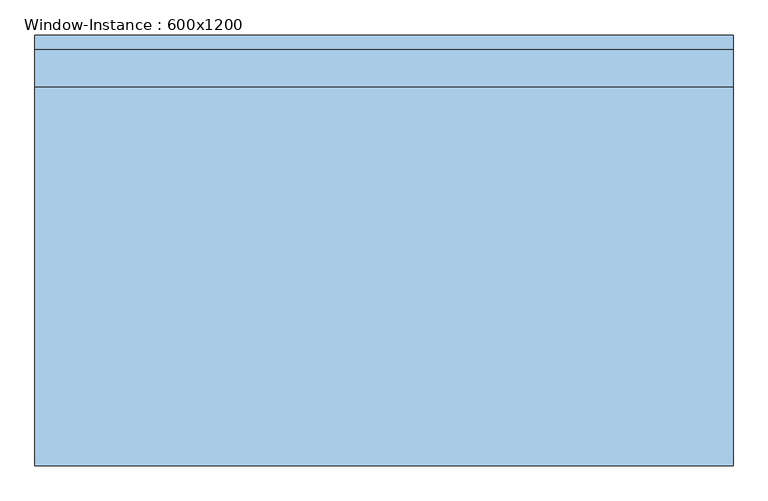
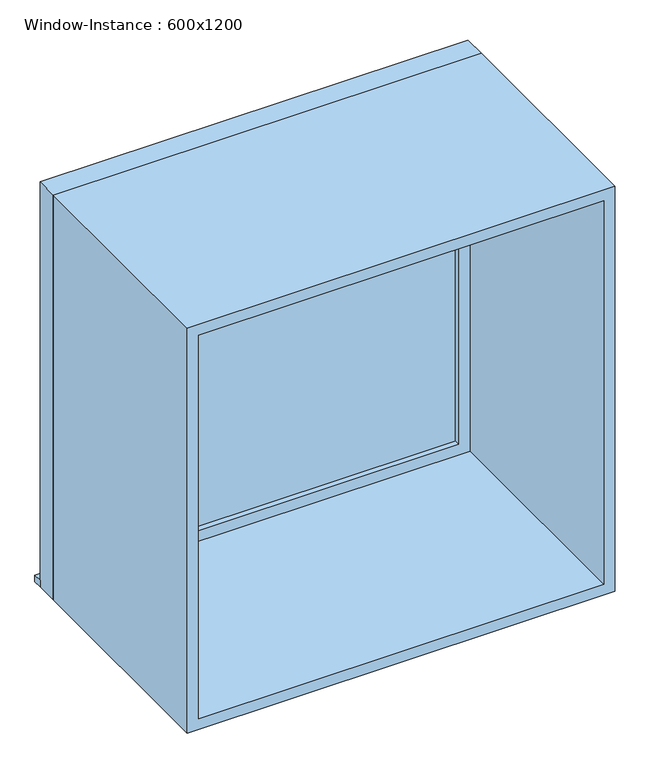
"""IFC4 building model written with IfcOpenShell, lengths in millimetres: window geometry, Window-Instance : 600x1200."""

import ifcopenshell
import ifcopenshell.guid

model = None  # the IFC model being written
_history = None  # IfcOwnerHistory: only IFC2X3 demands one
_inside = {}  # id of a spatial element -> (the spatial element, [elements in it])
_under = {}  # id of a project, library or spatial element -> (it, [spatial elements below it])
_declared = {}  # id of a project -> (the project, [libraries it declares])
_typed = {}  # id of a type object -> (the type object, [elements of that type])
_made_of = {}  # id of a material, layer set ... -> (it, [elements and type objects made of it])


def new_model(schema):
    """Start an empty IFC model of exactly this schema.

    Asked for "IFC4X3", IfcOpenShell would pick the latest addendum, in which some entities
    have other attributes; the version numbers below select the first issue.
    IFC2X3 requires an IfcOwnerHistory on every rooted entity: one is made here for all.
    """
    global model, _history
    if schema == "IFC4X3":
        model = ifcopenshell.file(schema_version=(4, 3, 0, 0))
    else:
        model = ifcopenshell.file(schema=schema)
    _inside.clear()
    _under.clear()
    _declared.clear()
    _typed.clear()
    _made_of.clear()
    _history = None
    if model.schema == "IFC2X3":
        org = make("IfcOrganization", Name="unknown")
        user = make(
            "IfcPersonAndOrganization",
            ThePerson=make("IfcPerson", FamilyName="unknown"),
            TheOrganization=org,
        )
        app = make(
            "IfcApplication",
            ApplicationDeveloper=org,
            Version="unknown",
            ApplicationFullName="unknown",
            ApplicationIdentifier="unknown",
        )
        _history = make(
            "IfcOwnerHistory",
            OwningUser=user,
            OwningApplication=app,
            ChangeAction="ADDED",
            CreationDate=0,
        )
    return model


def make(cls, **values):
    """One entity of the class cls with the attributes given. An attribute that is None is left unset."""
    return model.create_entity(
        cls, **{name: value for name, value in values.items() if value is not None}
    )


def rooted(cls, **values):
    """An entity with a GlobalId (a new one), such as an element, a storey or a relation."""
    return make(cls, GlobalId=ifcopenshell.guid.new(), OwnerHistory=_history, **values)


def si_unit(unit_type, name, prefix=None):
    """IfcSIUnit, for example si_unit("LENGTHUNIT", "METRE", prefix="MILLI")."""
    return make("IfcSIUnit", UnitType=unit_type, Prefix=prefix, Name=name)


def assignment(units):
    """IfcUnitAssignment: the units of a project."""
    return None if units is None else make("IfcUnitAssignment", Units=units)


def point(xyz):
    """IfcCartesianPoint."""
    return None if xyz is None else make("IfcCartesianPoint", Coordinates=xyz)


def direction(xyz):
    """IfcDirection."""
    return None if xyz is None else make("IfcDirection", DirectionRatios=xyz)


def frame(location, z_axis=None, x_axis=None):
    """IfcAxis2Placement3D, a coordinate frame: its origin and axes. An axis left out is left unset."""
    return make(
        "IfcAxis2Placement3D",
        Location=point(location),
        Axis=direction(z_axis),
        RefDirection=direction(x_axis),
    )


def origin():
    """The frame at (0, 0, 0) with its axes left unset."""
    return frame((0.0, 0.0, 0.0))


def place(relative_to, where):
    """IfcLocalPlacement: puts the frame where relative to a parent placement (None: the world)."""
    return make(
        "IfcLocalPlacement", PlacementRelTo=relative_to, RelativePlacement=where
    )


def context(
    kind, dimensions, precision=None, world=None, true_north=None, identifier=None
):
    """IfcGeometricRepresentationContext, for example the 3D "Model" context."""
    return make(
        "IfcGeometricRepresentationContext",
        ContextIdentifier=identifier,
        ContextType=kind,
        CoordinateSpaceDimension=dimensions,
        Precision=precision,
        WorldCoordinateSystem=world,
        TrueNorth=true_north,
    )


def project(units=None, contexts=None):
    """IfcProject with its units and contexts."""
    return rooted(
        "IfcProject",
        Name="project",
        RepresentationContexts=contexts,
        UnitsInContext=assignment(units),
    )


def spatial(cls, under=None, at=None, **own):
    """A site, building, storey or space (cls), placed at a placement, below another one or the project."""
    s = rooted(cls, ObjectPlacement=at, **own)
    if under is not None:
        _under.setdefault(under.id(), (under, []))[1].append(s)
    return s


def polyline(points):
    """IfcPolyline through the points."""
    return make("IfcPolyline", Points=[point(p) for p in points])


def outline(outer, holes=None, kind="AREA"):
    """IfcArbitraryClosedProfileDef: a profile drawn as a closed curve; with holes, ...WithVoids."""
    if holes is None:
        return make("IfcArbitraryClosedProfileDef", ProfileType=kind, OuterCurve=outer)
    return make(
        "IfcArbitraryProfileDefWithVoids",
        ProfileType=kind,
        OuterCurve=outer,
        InnerCurves=holes,
    )


def extrude(swept, where, along, depth):
    """IfcExtrudedAreaSolid: the profile swept, set in the frame where, extruded along a direction by depth."""
    return make(
        "IfcExtrudedAreaSolid",
        SweptArea=swept,
        Position=where,
        ExtrudedDirection=direction(along),
        Depth=depth,
    )


def shape(context_of_items, identifier, shape_type, items):
    """IfcShapeRepresentation: the items that make up one representation, for example the "Body"."""
    return make(
        "IfcShapeRepresentation",
        ContextOfItems=context_of_items,
        RepresentationIdentifier=identifier,
        RepresentationType=shape_type,
        Items=items,
    )


def source(mapping_origin, context_of_items, identifier, shape_type, items):
    """IfcRepresentationMap: a shape defined once, which mapped items show again and again."""
    return make(
        "IfcRepresentationMap",
        MappingOrigin=mapping_origin,
        MappedRepresentation=shape(context_of_items, identifier, shape_type, items),
    )


def transform(
    local_origin,
    x_axis=None,
    y_axis=None,
    z_axis=None,
    scale=None,
    scale2=None,
    scale3=None,
    uniform=True,
):
    """IfcCartesianTransformationOperator3D, or its non-uniform kind. x_axis, y_axis, z_axis: its Axis1, 2, 3."""
    if uniform:
        return make(
            "IfcCartesianTransformationOperator3D",
            Axis1=direction(x_axis),
            Axis2=direction(y_axis),
            LocalOrigin=point(local_origin),
            Scale=scale,
            Axis3=direction(z_axis),
        )
    return make(
        "IfcCartesianTransformationOperator3DnonUniform",
        Axis1=direction(x_axis),
        Axis2=direction(y_axis),
        LocalOrigin=point(local_origin),
        Scale=scale,
        Axis3=direction(z_axis),
        Scale2=scale2,
        Scale3=scale3,
    )


def mapped(mapping_source, mapping_target):
    """IfcMappedItem: shows the shape of a source again, moved by a transform."""
    return make(
        "IfcMappedItem", MappingSource=mapping_source, MappingTarget=mapping_target
    )


def made_of(thing, what):
    """Note that an element or type object is made of a material, layer set ...; save() writes the relation."""
    if what is not None:
        _made_of.setdefault(what.id(), (what, []))[1].append(thing)
    return thing


def element(
    cls,
    number,
    at=None,
    inside=None,
    cuts=None,
    type_object=None,
    material=None,
    context=None,
    identifier="Body",
    shape_type=None,
    held_by="IfcProductDefinitionShape",
    body=None,
    shapes=None,
    **own,
):
    """One element of the class cls, such as IfcWall. Its Tag is "e" and its number.

    at: its placement. inside: the storey or other place that contains it. cuts: it is an
    opening in that element (IfcRelVoidsElement). A single representation is given by context,
    identifier, shape_type and body (its items); several are given by shapes. held_by: the class
    of the entity that holds the representations. save() writes the other relations.
    """
    e = rooted(cls, Tag="e%d" % number, ObjectPlacement=at, **own)
    if body is not None:
        shapes = [shape(context, identifier, shape_type, body)]
    if shapes is not None:
        e.Representation = make(held_by, Representations=shapes)
    if inside is not None:
        _inside.setdefault(inside.id(), (inside, []))[1].append(e)
    if cuts is not None:
        rooted(
            "IfcRelVoidsElement", RelatingBuildingElement=cuts, RelatedOpeningElement=e
        )
    if type_object is not None:
        _typed.setdefault(type_object.id(), (type_object, []))[1].append(e)
    return made_of(e, material)


def aggregate(whole, parts):
    """IfcRelAggregates: a whole, such as a stair, and the parts it consists of."""
    return rooted("IfcRelAggregates", RelatingObject=whole, RelatedObjects=parts)


def save(model, path):
    """Write the relations noted so far, then the file.

    IfcRelAggregates (storeys below a building ...), IfcRelContainedInSpatialStructure (elements
    in a storey), IfcRelDefinesByType, IfcRelAssociatesMaterial and IfcRelDeclares: one each for
    every whole, place, type object, material and project.
    """
    for whole, parts in _under.values():
        aggregate(whole, parts)
    for where, things in _inside.values():
        rooted(
            "IfcRelContainedInSpatialStructure",
            RelatedElements=things,
            RelatingStructure=where,
        )
    for kind, things in _typed.values():
        rooted("IfcRelDefinesByType", RelatedObjects=things, RelatingType=kind)
    for what, things in _made_of.values():
        rooted("IfcRelAssociatesMaterial", RelatedObjects=things, RelatingMaterial=what)
    for by, libraries in _declared.values():
        rooted("IfcRelDeclares", RelatingContext=by, RelatedDefinitions=libraries)
    model.write(path)


def window_instance_600x1200_c70fa3c9(model_context):
    return source(origin(), model_context, "Body", "SweptSolid", [
        extrude(outline(polyline([(-638.1, 382.9), (561.9, 382.9), (561.9, 357.5), (-638.1, 357.5), (-638.1, 382.9)])), frame((0.0, 0.0, 900.0), z_axis=(0.0, 0.0, 1.0), x_axis=(1.0, 0.0, 0.0)), (0.0, 0.0, 1.0), 19.05),
        extrude(outline(polyline([(498.4, 308.925), (-574.6, 308.925), (-574.6, 321.625), (498.4, 321.625), (498.4, 308.925)])), frame((0.0, 0.0, 963.5), z_axis=(0.0, 0.0, 1.0), x_axis=(1.0, 0.0, 0.0)), (0.0, 0.0, 1.0), 1073.0),
        extrude(outline(polyline([(2080.95, -619.05), (919.05, -619.05), (919.05, 542.85), (2080.95, 542.85), (2080.95, -619.05)]), holes=[polyline([(2036.5, -574.6), (2036.5, 498.4), (963.5, 498.4), (963.5, -574.6), (2036.5, -574.6)])]), frame((0.0, 293.05, 0.0), z_axis=(0.0, 1.0, 0.0), x_axis=(0.0, 0.0, 1.0)), (0.0, 0.0, 1.0), 44.45),
        extrude(outline(polyline([(2100.0, -638.1), (900.0, -638.1), (900.0, 561.9), (2100.0, 561.9), (2100.0, -638.1)]), holes=[polyline([(2068.25, -606.35), (2068.25, 530.15), (931.75, 530.15), (931.75, -606.35), (2068.25, -606.35)])]), frame((0.0, -357.5, 0.0), z_axis=(0.0, 1.0, 0.0), x_axis=(0.0, 0.0, 1.0)), (0.0, 0.0, 1.0), 650.55),
        extrude(outline(polyline([(2100.0, 561.9), (2100.0, -638.1), (900.0, -638.1), (900.0, 561.9), (2100.0, 561.9)]), holes=[polyline([(2080.95, 542.85), (919.05, 542.85), (919.05, -619.05), (2080.95, -619.05), (2080.95, 542.85)])]), frame((0.0, 293.05, 0.0), z_axis=(0.0, 1.0, 0.0), x_axis=(0.0, 0.0, 1.0)), (0.0, 0.0, 1.0), 64.45),
    ])


if __name__ == "__main__":
    model = new_model("IFC4")
    model_context = context("Model", 3, world=origin())
    ifc_project = project(units=[si_unit("LENGTHUNIT", "METRE", prefix="MILLI")], contexts=[model_context])
    site = spatial("IfcSite", under=ifc_project)
    building = spatial("IfcBuilding", under=site)
    placement = place(None, origin())
    window_instance_600x1200_shape = window_instance_600x1200_c70fa3c9(model_context)
    element("IfcWindow", 1, ObjectType="Window-Instance : 600x1200", at=placement, inside=building, context=model_context, shape_type="MappedRepresentation", body=[
        mapped(window_instance_600x1200_shape, transform((0.0, 0.0, 0.0), x_axis=(1.0, 0.0, 0.0), y_axis=(0.0, 1.0, 0.0), z_axis=(0.0, 0.0, 1.0))),
    ])
    save(model, "model.ifc")

# Revit data of these elements
# Type "Window-Instance : 600x1200"
#   Type Mark = "7"
#   Construction Type Id = "GSP4R"
#   Assembly Code = "B2020100"
#   Analytic Construction = "1/8 in Pilkington single glazing"
#   Visual Light Transmittance = 0.9
#   Thermal Resistance (R) = 0.149095 (m²·K)/W
#   Solar Heat Gain Coefficient = 0.86
#   Heat Transfer Coefficient (U) = 6.70716 W/(m²·K)
#   Height [instance default] = 1200 mm
#   Default Sill Height = 900 mm
#   Width [instance default] = 600 mm
#   Window Inset = 20 mm
#   Glass Pane Material = WW-EC-GL-Storefront
#   Sash Material = WW-EC-RGB-White
#   Wall Closure = (empty or 0)
# Element 1 (IfcWindow, "Window-Instance : 600x1200")
#   Width = 1200 mm
#   Materials on its faces: "WW-EC-RGB-White", "WW-EC-GL-Storefront"
# Materials
#   "WW-EC-GL-Storefront": class "Glass", colour RGB 236 240 239, transparency 0.85, Description = "Storefront Glass", Cost = 0
#   "WW-EC-RGB-White": class "Generic", colour RGB 255 255 255, transparency 0, Comments = "If region requests off-white, swith asset color to RGB 231-228-220", Description = "Generic Color", Cost = 0
